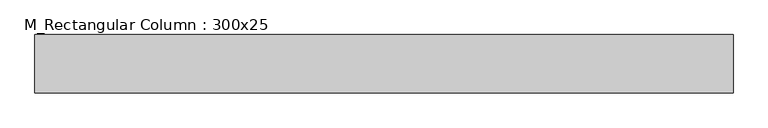
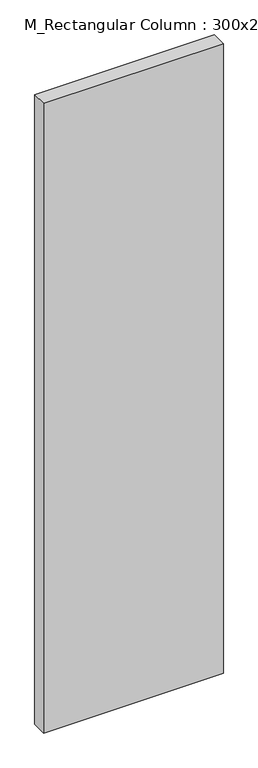
"""IFC4 building model written with IfcOpenShell, lengths in millimetres: column geometry, M_Rectangular Column : 300x25."""

from ifc_helpers import new_model, si_unit, frame, origin, place, context, project, spatial, polyline, outline, extrude, source, transform, mapped, element, save


def m_rectangular_column_300x25_b7e4e278(model_context):
    return source(origin(), model_context, "Body", "SweptSolid", [
        extrude(outline(polyline([(1500.0, 125.0), (1500.0, -125.0), (-1500.0, -125.0), (-1500.0, 125.0), (1500.0, 125.0)])), frame((0.0, 0.0, -3200.0), z_axis=(0.0, 0.0, 1.0), x_axis=(1.0, 0.0, 0.0)), (0.0, 0.0, 1.0), 11100.0),
    ])


if __name__ == "__main__":
    model = new_model("IFC4")
    model_context = context("Model", 3, world=origin())
    ifc_project = project(units=[si_unit("LENGTHUNIT", "METRE", prefix="MILLI")], contexts=[model_context])
    site = spatial("IfcSite", under=ifc_project)
    building = spatial("IfcBuilding", under=site)
    placement = place(None, origin())
    m_rectangular_column_300x25_shape = m_rectangular_column_300x25_b7e4e278(model_context)
    element("IfcColumn", 1, ObjectType="M_Rectangular Column : 300x25", at=placement, inside=building, context=model_context, shape_type="MappedRepresentation", body=[
        mapped(m_rectangular_column_300x25_shape, transform((0.0, 0.0, 0.0), x_axis=(1.0, 0.0, 0.0), y_axis=(0.0, 1.0, 0.0), z_axis=(0.0, 0.0, 1.0))),
    ])
    save(model, "model.ifc")

# Revit data of these elements
# Type "M_Rectangular Column : 300x25"
#   Depth = 25 cm
#   Offset Base = 0 cm
#   Offset Top = 0 cm
#   Width = 300 cm
#   Material = none
